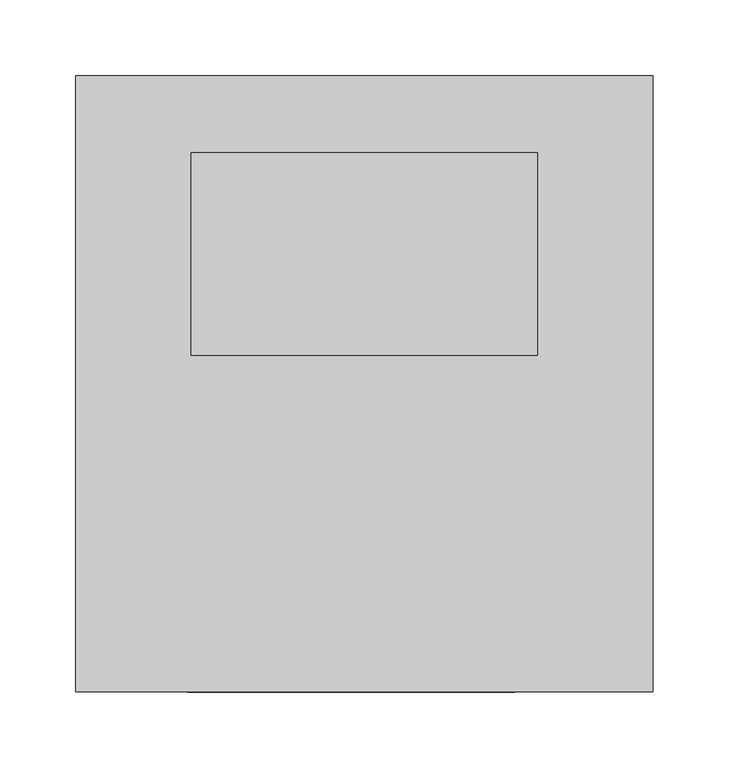
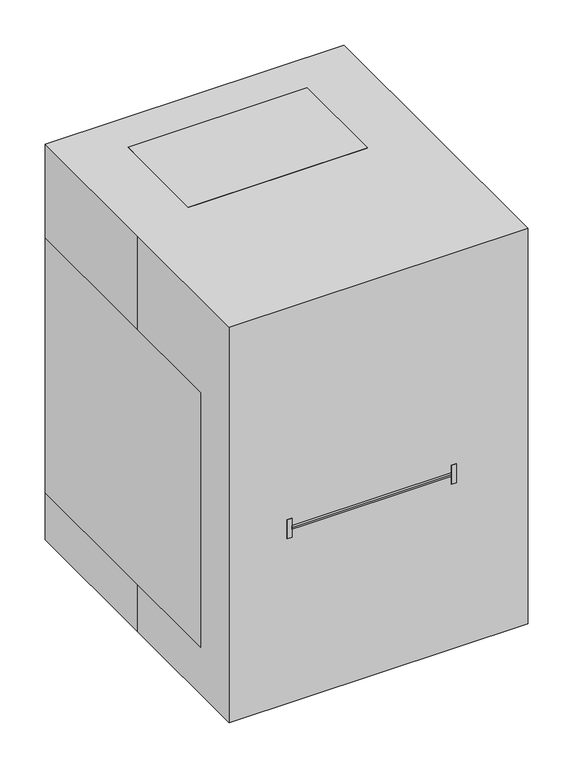
"""IFC4 building model written with IfcOpenShell, lengths in millimetres: proxy geometry, D4500 - Furnace, Laboratory, Dental, Burnout : D4500 - Furnace, Laboratory, Dental, Burnout."""

from ifc_helpers import new_model, si_unit, point, frame, frame_2d, origin, origin_with_axes, place, context, project, spatial, polyline, circle_curve, ellipse_curve, trimmed, segment, composite_curve, outline, extrude, source, transform, mapped, element, save
from ifc_brep_helpers import plane_surface, revolved_surface, advanced_brep


def specialty_equipment_c4cd605c(model_context):
    return source(origin(), model_context, "Body", "SolidModel", [
        extrude(outline(polyline([(0.0, -25.5914377), (0.0, 0.0), (12.6999999, 0.0), (12.6999999, -25.5914377), (0.0, -25.5914377)])), frame((58.817219, -9.8927789, 446.2580582), z_axis=(0.0, 0.18428853505018944, 0.9828721869343212), x_axis=(0.0, 0.9828721869343212, -0.18428853505018944)), (0.0, 0.0, 1.0), 12.7),
        extrude(outline(polyline([(0.0, -39.4493307), (0.0, 0.0), (12.7, 0.0), (12.7, -39.4493307), (0.0, -39.4493307)])), frame((58.817219, -5.1590339, 473.1988265), z_axis=(0.0, 0.18428853505018944, 0.9828721869343212), x_axis=(0.0, 0.9828721869343212, -0.18428853505018944)), (0.0, 0.0, 1.0), 12.7),
        advanced_brep(
        [(-33.7035425, 19.6808212, 515.5977131), (-61.832781, 19.6808212, 515.5977131), (-61.832781, 19.6808212, 502.8977131), (-33.7035425, 19.6808212, 502.8977131), (-33.7035425, 15.7120712, 515.5977131), (-61.832781, 15.7120712, 515.5977131), (-61.832781, 13.3308212, 502.8977131), (-33.7035425, 13.3308212, 502.8977131), (10.7464575, 19.6808212, 515.5977131), (-17.382781, 19.6808212, 515.5977131), (-17.382781, 19.6808212, 502.8977131), (10.7464575, 19.6808212, 502.8977131), (10.7464575, 15.7120712, 515.5977131), (-17.382781, 15.7120712, 515.5977131), (-17.382781, 13.3308212, 502.8977131), (10.7464575, 13.3308212, 502.8977131), (86.9464575, 19.6808212, 515.5977131), (58.817219, 19.6808212, 515.5977131), (58.817219, 19.6808212, 502.8977131), (86.9464575, 19.6808212, 502.8977131), (86.9464575, 15.7120712, 515.5977131), (58.817219, 15.7120712, 515.5977131), (58.817219, 13.3308212, 502.8977131), (86.9464575, 13.3308212, 502.8977131), (-81.3285425, 19.6808212, 515.5977131), (-98.425, 19.6808212, 515.5977131), (-98.425, 19.6808212, 502.8977131), (-81.3285425, 19.6808212, 502.8977131), (-81.3285425, 15.7120712, 515.5977131), (-98.425, 15.7120712, 515.5977131), (-98.425, 13.3308212, 502.8977131), (-81.3285425, 13.3308212, 502.8977131), (-1.1880744, 19.9716696, 476.932238), (11.5119256, 19.9716696, 476.932238), (-1.1880744, 8.4622946, 476.932238), (5.1619256, 7.2716696, 470.582238), (11.5119256, 8.4622946, 476.932238), (11.148763, 3.3029196, 449.4155713), (-0.8249118, 3.3029196, 449.4155713), (-1.1880744, 16.0029196, 451.532238), (11.5119256, 16.0029196, 451.532238), (-1.1880744, 3.6997946, 451.532238), (11.5119256, 3.6997946, 451.532238), (-13.5268228, 5.6841696, 462.1155713), (-19.8099793, 5.6841696, 462.1155713), (-23.0184011, 18.3841696, 467.6339938), (-10.3184011, 18.3841696, 467.6339938), (-23.0184011, 6.7188738, 467.6339938), (-10.3184011, 6.7188738, 467.6339938), (-38.9268228, 5.6841696, 462.1155713), (-45.2099793, 5.6841696, 462.1155713), (-48.4184011, 19.9716696, 467.6339938), (-35.7184011, 19.9716696, 467.6339938), (-48.4184011, 6.7188738, 467.6339938), (-35.7184011, 6.7188738, 467.6339938), (-64.3268228, 5.6841696, 462.1155713), (-70.6099793, 5.6841696, 462.1155713), (-73.8184011, 19.9716696, 467.6339938), (-61.1184011, 19.9716696, 467.6339938), (-73.8184011, 6.7188738, 467.6339938), (-61.1184011, 6.7188738, 467.6339938), (-86.5509752, 5.6841696, 462.1155713), (-92.8341316, 5.6841696, 462.1155713), (-96.0425534, 17.4344988, 467.6339938), (-83.3425534, 17.4344988, 467.6339938), (-96.0425534, 6.7188738, 467.6339938), (-83.3425534, 6.7188738, 467.6339938), (114.3, 152.4, 533.4), (-114.3, 152.4, 533.4), (-114.3, 19.05, 533.4), (114.3, 19.05, 533.4), (114.3, 152.4, 431.8), (114.3, 0.0, 431.8), (-114.3, 0.0, 431.8), (-114.3, 152.4, 431.8)],
        [
            (0, 1),
            (1, 2),
            (2, 3),
            (3, 0),
            (0, 4),
            (4, 5),
            (5, 1),
            (5, 6),
            (6, 2),
            (6, 7),
            (7, 3),
            (7, 4),
            (8, 9),
            (9, 10),
            (10, 11),
            (11, 8),
            (8, 12),
            (12, 13),
            (13, 9),
            (13, 14),
            (14, 10),
            (14, 15),
            (15, 11),
            (15, 12),
            (16, 17),
            (17, 18),
            (18, 19),
            (19, 16),
            (16, 20),
            (20, 21),
            (21, 17),
            (21, 22),
            (22, 18),
            (22, 23),
            (23, 19),
            (23, 20),
            (24, 25),
            (25, 26),
            (26, 27),
            (27, 24),
            (24, 28),
            (28, 29),
            (29, 25),
            (29, 30),
            (30, 26),
            (30, 31),
            (31, 27),
            (31, 28),
            (32, 33, circle_curve(frame((5.1619256, 19.9716696, 476.932238), z_axis=(0.0, -1.0, 0.0), x_axis=(1.0, 0.0, 0.0)), 6.35)),
            (33, 32, circle_curve(frame((5.1619256, 19.9716696, 476.932238), z_axis=(0.0, -1.0, 0.0), x_axis=(1.0, 0.0, 0.0)), 6.35)),
            (32, 34),
            (34, 35, ellipse_curve(frame((5.1619256, 8.4622946, 476.932238), z_axis=(0.0, -0.9828721869343219, 0.18428853505018564), x_axis=(0.0, -0.18428853505018514, -0.9828721869343221)), 6.4606569, 6.35)),
            (35, 36, ellipse_curve(frame((5.1619256, 8.4622946, 476.932238), z_axis=(0.0, -0.9828721869343219, 0.18428853505018564), x_axis=(0.0, -0.18428853505018514, -0.9828721869343221)), 6.4606569, 6.35)),
            (36, 33),
            (36, 34, ellipse_curve(frame((5.1619256, 8.4622946, 476.932238), z_axis=(0.0, -0.9828721869343219, 0.18428853505018564), x_axis=(0.0, -0.18428853505018514, -0.9828721869343221)), 6.4606569, 6.35)),
            (37, 38, circle_curve(frame((5.1619256, 3.3029196, 451.532238), z_axis=(0.0, 1.0, 0.0), x_axis=(1.0, 0.0, 0.0)), 6.35)),
            (38, 37),
            (39, 40, circle_curve(frame((5.1619256, 16.0029196, 451.532238), z_axis=(0.0, -1.0, 0.0), x_axis=(1.0, 0.0, 0.0)), 6.35)),
            (40, 39, circle_curve(frame((5.1619256, 16.0029196, 451.532238), z_axis=(0.0, -1.0, 0.0), x_axis=(1.0, 0.0, 0.0)), 6.35)),
            (39, 41),
            (41, 38, ellipse_curve(frame((5.1619256, 3.6997946, 451.532238), z_axis=(0.0, -0.9828721869343219, 0.18428853505018564), x_axis=(0.0, -0.18428853505018514, -0.9828721869343221)), 6.4606569, 6.35)),
            (37, 42, ellipse_curve(frame((5.1619256, 3.6997946, 451.532238), z_axis=(0.0, -0.9828721869343219, 0.18428853505018564), x_axis=(0.0, -0.18428853505018514, -0.9828721869343221)), 6.4606569, 6.35)),
            (42, 40),
            (42, 41, ellipse_curve(frame((5.1619256, 3.6997946, 451.532238), z_axis=(0.0, -0.9828721869343219, 0.18428853505018564), x_axis=(0.0, -0.18428853505018514, -0.9828721869343221)), 6.4606569, 6.35)),
            (43, 44, circle_curve(frame((-16.6684011, 5.6841696, 467.6339938), z_axis=(0.0, 1.0, 0.0), x_axis=(1.0, 0.0, 0.0)), 6.35)),
            (44, 43),
            (45, 46, circle_curve(frame((-16.6684011, 18.3841696, 467.6339938), z_axis=(0.0, -1.0, 0.0), x_axis=(1.0, 0.0, 0.0)), 6.35)),
            (46, 45, circle_curve(frame((-16.6684011, 18.3841696, 467.6339938), z_axis=(0.0, -1.0, 0.0), x_axis=(1.0, 0.0, 0.0)), 6.35)),
            (45, 47),
            (47, 44, ellipse_curve(frame((-16.6684011, 6.7188738, 467.6339938), z_axis=(0.0, -0.9828721869343219, 0.18428853505018564), x_axis=(0.0, -0.18428853505018514, -0.9828721869343221)), 6.4606569, 6.35)),
            (43, 48, ellipse_curve(frame((-16.6684011, 6.7188738, 467.6339938), z_axis=(0.0, -0.9828721869343219, 0.18428853505018564), x_axis=(0.0, -0.18428853505018514, -0.9828721869343221)), 6.4606569, 6.35)),
            (48, 46),
            (48, 47, ellipse_curve(frame((-16.6684011, 6.7188738, 467.6339938), z_axis=(0.0, -0.9828721869343219, 0.18428853505018564), x_axis=(0.0, -0.18428853505018514, -0.9828721869343221)), 6.4606569, 6.35)),
            (49, 50, circle_curve(frame((-42.0684011, 5.6841696, 467.6339938), z_axis=(0.0, 1.0, 0.0), x_axis=(1.0, 0.0, 0.0)), 6.35)),
            (50, 49),
            (51, 52, circle_curve(frame((-42.0684011, 19.9716696, 467.6339938), z_axis=(0.0, -1.0, 0.0), x_axis=(1.0, 0.0, 0.0)), 6.35)),
            (52, 51, circle_curve(frame((-42.0684011, 19.9716696, 467.6339938), z_axis=(0.0, -1.0, 0.0), x_axis=(1.0, 0.0, 0.0)), 6.35)),
            (51, 53),
            (53, 50, ellipse_curve(frame((-42.0684011, 6.7188738, 467.6339938), z_axis=(0.0, -0.9828721869343219, 0.18428853505018564), x_axis=(0.0, -0.18428853505018514, -0.9828721869343221)), 6.4606569, 6.35)),
            (49, 54, ellipse_curve(frame((-42.0684011, 6.7188738, 467.6339938), z_axis=(0.0, -0.9828721869343219, 0.18428853505018564), x_axis=(0.0, -0.18428853505018514, -0.9828721869343221)), 6.4606569, 6.35)),
            (54, 52),
            (54, 53, ellipse_curve(frame((-42.0684011, 6.7188738, 467.6339938), z_axis=(0.0, -0.9828721869343219, 0.18428853505018564), x_axis=(0.0, -0.18428853505018514, -0.9828721869343221)), 6.4606569, 6.35)),
            (55, 56, circle_curve(frame((-67.4684011, 5.6841696, 467.6339938), z_axis=(0.0, 1.0, 0.0), x_axis=(1.0, 0.0, 0.0)), 6.35)),
            (56, 55),
            (57, 58, circle_curve(frame((-67.4684011, 19.9716696, 467.6339938), z_axis=(0.0, -1.0, 0.0), x_axis=(1.0, 0.0, 0.0)), 6.35)),
            (58, 57, circle_curve(frame((-67.4684011, 19.9716696, 467.6339938), z_axis=(0.0, -1.0, 0.0), x_axis=(1.0, 0.0, 0.0)), 6.35)),
            (57, 59),
            (59, 56, ellipse_curve(frame((-67.4684011, 6.7188738, 467.6339938), z_axis=(0.0, -0.9828721869343219, 0.18428853505018564), x_axis=(0.0, -0.18428853505018514, -0.9828721869343221)), 6.4606569, 6.35)),
            (55, 60, ellipse_curve(frame((-67.4684011, 6.7188738, 467.6339938), z_axis=(0.0, -0.9828721869343219, 0.18428853505018564), x_axis=(0.0, -0.18428853505018514, -0.9828721869343221)), 6.4606569, 6.35)),
            (60, 58),
            (60, 59, ellipse_curve(frame((-67.4684011, 6.7188738, 467.6339938), z_axis=(0.0, -0.9828721869343219, 0.18428853505018564), x_axis=(0.0, -0.18428853505018514, -0.9828721869343221)), 6.4606569, 6.35)),
            (61, 62, circle_curve(frame((-89.6925534, 5.6841696, 467.6339938), z_axis=(0.0, 1.0, 0.0), x_axis=(1.0, 0.0, 0.0)), 6.35)),
            (62, 61),
            (63, 64, circle_curve(frame((-89.6925534, 17.4344988, 467.6339938), z_axis=(0.0, -1.0, 0.0), x_axis=(1.0, 0.0, 0.0)), 6.35)),
            (64, 63, circle_curve(frame((-89.6925534, 17.4344988, 467.6339938), z_axis=(0.0, -1.0, 0.0), x_axis=(1.0, 0.0, 0.0)), 6.35)),
            (63, 65),
            (65, 62, ellipse_curve(frame((-89.6925534, 6.7188738, 467.6339938), z_axis=(0.0, -0.9828721869343219, 0.18428853505018564), x_axis=(0.0, -0.18428853505018514, -0.9828721869343221)), 6.4606569, 6.35)),
            (61, 66, ellipse_curve(frame((-89.6925534, 6.7188738, 467.6339938), z_axis=(0.0, -0.9828721869343219, 0.18428853505018564), x_axis=(0.0, -0.18428853505018514, -0.9828721869343221)), 6.4606569, 6.35)),
            (66, 64),
            (66, 65, ellipse_curve(frame((-89.6925534, 6.7188738, 467.6339938), z_axis=(0.0, -0.9828721869343219, 0.18428853505018564), x_axis=(0.0, -0.18428853505018514, -0.9828721869343221)), 6.4606569, 6.35)),
            (67, 68),
            (68, 69),
            (69, 70),
            (70, 67),
            (71, 72),
            (72, 73),
            (73, 74),
            (74, 71),
            (67, 71),
            (74, 68),
            (73, 69),
            (72, 70),
        ],
        [
            plane_surface(frame((-61.832781, 19.6808212, 515.5977131), z_axis=(0.0, -1.0, 0.0), x_axis=(1.0, 0.0, 0.0))),
            plane_surface(frame((-33.7035425, 13.3308212, 515.5977131), z_axis=(0.0, 0.0, -1.0), x_axis=(0.0, 1.0, 0.0))),
            plane_surface(frame((-61.832781, 13.3308212, 515.5977131), z_axis=(1.0, 0.0, 0.0), x_axis=(0.0, 1.0, 0.0))),
            plane_surface(frame((-61.832781, 13.3308212, 502.8977131), z_axis=(0.0, 0.0, 1.0), x_axis=(0.0, 1.0, 0.0))),
            plane_surface(frame((-33.7035425, 13.3308212, 502.8977131), z_axis=(-1.0, 0.0, 0.0), x_axis=(0.0, 1.0, 0.0))),
            plane_surface(frame((-17.382781, 19.6808212, 515.5977131), z_axis=(0.0, -1.0, 0.0), x_axis=(1.0, 0.0, 0.0))),
            plane_surface(frame((10.7464575, 13.3308212, 515.5977131), z_axis=(0.0, 0.0, -1.0), x_axis=(0.0, 1.0, 0.0))),
            plane_surface(frame((-17.382781, 13.3308212, 515.5977131), z_axis=(1.0, 0.0, 0.0), x_axis=(0.0, 1.0, 0.0))),
            plane_surface(frame((-17.382781, 13.3308212, 502.8977131), z_axis=(0.0, 0.0, 1.0), x_axis=(0.0, 1.0, 0.0))),
            plane_surface(frame((10.7464575, 13.3308212, 502.8977131), z_axis=(-1.0, 0.0, 0.0), x_axis=(0.0, 1.0, 0.0))),
            plane_surface(frame((58.817219, 19.6808212, 515.5977131), z_axis=(0.0, -1.0, 0.0), x_axis=(1.0, 0.0, 0.0))),
            plane_surface(frame((86.9464575, 13.3308212, 515.5977131), z_axis=(0.0, 0.0, -1.0), x_axis=(0.0, 1.0, 0.0))),
            plane_surface(frame((58.817219, 13.3308212, 515.5977131), z_axis=(1.0, 0.0, 0.0), x_axis=(0.0, 1.0, 0.0))),
            plane_surface(frame((58.817219, 13.3308212, 502.8977131), z_axis=(0.0, 0.0, 1.0), x_axis=(0.0, 1.0, 0.0))),
            plane_surface(frame((86.9464575, 13.3308212, 502.8977131), z_axis=(-1.0, 0.0, 0.0), x_axis=(0.0, 1.0, 0.0))),
            plane_surface(frame((-109.457781, 19.6808212, 515.5977131), z_axis=(0.0, -1.0, 0.0), x_axis=(1.0, 0.0, 0.0))),
            plane_surface(frame((-81.3285425, 13.3308212, 515.5977131), z_axis=(0.0, 0.0, -1.0), x_axis=(0.0, 1.0, 0.0))),
            plane_surface(frame((-98.425, 13.3308212, 515.5977131), z_axis=(1.0, 0.0, 0.0), x_axis=(0.0, 1.0, 0.0))),
            plane_surface(frame((-98.425, 13.3308212, 502.8977131), z_axis=(0.0, 0.0, 1.0), x_axis=(0.0, 1.0, 0.0))),
            plane_surface(frame((-81.3285425, 13.3308212, 502.8977131), z_axis=(-1.0, 0.0, 0.0), x_axis=(0.0, 1.0, 0.0))),
            plane_surface(frame((11.5119256, 19.9716696, 476.932238), z_axis=(0.0, -1.0, 0.0), x_axis=(0.0, 0.0, -1.0))),
            revolved_surface(polyline([(11.5119256, 7.271669599999999, 476.932238), (11.5119256, 19.9716696, 476.932238)]), (5.1619256, 19.9716696, 476.932238), (0.0, -1.0, 0.0)),
            revolved_surface(polyline([(11.5119256, 7.271669604437129, 476.932238), (11.5119256, 19.9716696, 476.932238)]), (5.1619256, 19.9716696, 476.932238), (0.0, -1.0, 0.0)),
            plane_surface(frame((11.5119256, 3.3029196, 451.532238), z_axis=(0.0, 1.0, 0.0), x_axis=(0.0, 0.0, 1.0))),
            plane_surface(frame((11.5119256, 16.0029196, 451.532238), z_axis=(0.0, -1.0, 0.0), x_axis=(0.0, 0.0, -1.0))),
            revolved_surface(polyline([(11.5119256, 2.5091696044371297, 451.532238), (11.5119256, 16.0029196, 451.532238)]), (5.1619256, 16.0029196, 451.532238), (0.0, -1.0, 0.0)),
            plane_surface(frame((-10.3184011, 5.6841696, 467.6339938), z_axis=(0.0, 1.0, 0.0), x_axis=(0.0, 0.0, 1.0))),
            plane_surface(frame((-10.3184011, 18.3841696, 467.6339938), z_axis=(0.0, -1.0, 0.0), x_axis=(0.0, 0.0, -1.0))),
            revolved_surface(polyline([(-10.3184011, 5.52824880443713, 467.6339938), (-10.3184011, 18.3841696, 467.6339938)]), (-16.6684011, 18.3841696, 467.6339938), (0.0, -1.0, 0.0)),
            plane_surface(frame((-35.7184011, 5.6841696, 467.6339938), z_axis=(0.0, 1.0, 0.0), x_axis=(0.0, 0.0, 1.0))),
            plane_surface(frame((-35.7184011, 19.9716696, 467.6339938), z_axis=(0.0, -1.0, 0.0), x_axis=(0.0, 0.0, -1.0))),
            revolved_surface(polyline([(-35.7184011, 5.52824880443713, 467.6339938), (-35.7184011, 19.9716696, 467.6339938)]), (-42.0684011, 19.9716696, 467.6339938), (0.0, -1.0, 0.0)),
            plane_surface(frame((-61.1184011, 5.6841696, 467.6339938), z_axis=(0.0, 1.0, 0.0), x_axis=(0.0, 0.0, 1.0))),
            plane_surface(frame((-61.1184011, 19.9716696, 467.6339938), z_axis=(0.0, -1.0, 0.0), x_axis=(0.0, 0.0, -1.0))),
            revolved_surface(polyline([(-61.11840109999999, 5.52824880443713, 467.6339938), (-61.11840109999999, 19.9716696, 467.6339938)]), (-67.4684011, 19.9716696, 467.6339938), (0.0, -1.0, 0.0)),
            plane_surface(frame((-83.3425534, 5.6841696, 467.6339938), z_axis=(0.0, 1.0, 0.0), x_axis=(0.0, 0.0, 1.0))),
            plane_surface(frame((-83.3425534, 17.4344988, 467.6339938), z_axis=(0.0, -1.0, 0.0), x_axis=(0.0, 0.0, -1.0))),
            revolved_surface(polyline([(-83.3425534, 5.52824880443713, 467.6339938), (-83.3425534, 17.4344988, 467.6339938)]), (-89.6925534, 17.4344988, 467.6339938), (0.0, -1.0, 0.0)),
            plane_surface(frame((0.0, 85.725, 533.4), z_axis=(0.0, 0.0, 1.0), x_axis=(-1.0, 0.0, 0.0))),
            plane_surface(frame((0.0, 76.2, 431.8), z_axis=(0.0, 0.0, -1.0), x_axis=(-1.0, 0.0, 0.0))),
            plane_surface(frame((0.0, 152.4, 431.8), z_axis=(0.0, 1.0, 0.0), x_axis=(-1.0, 0.0, 0.0))),
            plane_surface(frame((-114.3, 76.2, 431.8), z_axis=(-1.0, 0.0, 0.0), x_axis=(0.0, -1.0, 0.0))),
            plane_surface(frame((0.0, 0.0, 431.8), z_axis=(0.0, -0.9828721869343219, 0.18428853505018564), x_axis=(1.0, 0.0, 0.0))),
            plane_surface(frame((114.3, 76.2, 431.8), z_axis=(1.0, 0.0, 0.0), x_axis=(0.0, 1.0, 0.0))),
        ],
        [
            (0, [[1, 2, 3, 4]]),
            (1, [[-1, 5, 6, 7]]),
            (2, [[-2, -7, 8, 9]]),
            (3, [[-3, -9, 10, 11]]),
            (4, [[-4, -11, 12, -5]]),
            (5, [[13, 14, 15, 16]]),
            (6, [[-13, 17, 18, 19]]),
            (7, [[-14, -19, 20, 21]]),
            (8, [[-15, -21, 22, 23]]),
            (9, [[-16, -23, 24, -17]]),
            (10, [[25, 26, 27, 28]]),
            (11, [[-25, 29, 30, 31]]),
            (12, [[-26, -31, 32, 33]]),
            (13, [[-27, -33, 34, 35]]),
            (14, [[-28, -35, 36, -29]]),
            (15, [[37, 38, 39, 40]]),
            (16, [[-37, 41, 42, 43]]),
            (17, [[-38, -43, 44, 45]]),
            (18, [[-39, -45, 46, 47]]),
            (19, [[-40, -47, 48, -41]]),
            (20, [[49, 50]]),
            (21, [[-49, 51, 52, 53, 54]]),
            (22, [[-50, -54, 55, -51]]),
            (23, [[56, 57]]),
            (24, [[58, 59]]),
            (25, [[-58, 60, 61, -56, 62, 63]]),
            (25, [[-59, -63, 64, -60]]),
            (26, [[65, 66]]),
            (27, [[67, 68]]),
            (28, [[-67, 69, 70, -65, 71, 72]]),
            (28, [[-68, -72, 73, -69]]),
            (29, [[74, 75]]),
            (30, [[76, 77]]),
            (31, [[-76, 78, 79, -74, 80, 81]]),
            (31, [[-77, -81, 82, -78]]),
            (32, [[83, 84]]),
            (33, [[85, 86]]),
            (34, [[-85, 87, 88, -83, 89, 90]]),
            (34, [[-86, -90, 91, -87]]),
            (35, [[92, 93]]),
            (36, [[94, 95]]),
            (37, [[-94, 96, 97, -92, 98, 99]]),
            (37, [[-95, -99, 100, -96]]),
            (38, [[101, 102, 103, 104]]),
            (39, [[105, 106, 107, 108]]),
            (40, [[-101, 109, -108, 110]]),
            (41, [[-102, -110, -107, 111]]),
            (42, [[-103, -111, -106, 112], [-6, -12, -10, -8], [-18, -24, -22, -20], [-30, -36, -34, -32], [-42, -48, -46, -44], [-53, -52, -55], [-75, -79, -82, -80], [-84, -88, -91, -89], [-57, -61, -64, -62], [-93, -97, -100, -98], [-66, -70, -73, -71]]),
            (43, [[-104, -112, -105, -109]]),
        ],
    ),
        extrude(outline(polyline([(0.0, 140.2685872), (0.0, 165.6685872), (63.5, 165.6685872), (63.5, 127.5685872), (0.0, 140.2685872)])), frame((0.0, 139.7, 0.0), z_axis=(0.0, 1.0, 0.0), x_axis=(0.0, 0.0, 1.0)), (0.0, 0.0, 1.0), 38.1),
        extrude(outline(polyline([(0.0, -165.6685872), (0.0, -140.2685872), (63.5, -127.5685872), (63.5, -165.6685872), (0.0, -165.6685872)])), frame((0.0, 139.7, 0.0), z_axis=(0.0, 1.0, 0.0), x_axis=(0.0, 0.0, 1.0)), (0.0, 0.0, 1.0), 38.1),
        extrude(outline(polyline([(0.0, 140.2685872), (0.0, 165.6685872), (63.5, 165.6685872), (63.5, 127.5685872), (0.0, 140.2685872)])), frame((0.0, -114.3, 0.0), z_axis=(0.0, 1.0, 0.0), x_axis=(0.0, 0.0, 1.0)), (0.0, 0.0, 1.0), 38.1),
        extrude(outline(polyline([(0.0, -165.6685872), (0.0, -140.2685872), (63.5, -127.5685872), (63.5, -165.6685872), (0.0, -165.6685872)])), frame((0.0, -114.3, 0.0), z_axis=(0.0, 1.0, 0.0), x_axis=(0.0, 0.0, 1.0)), (0.0, 0.0, 1.0), 38.1),
        extrude(outline(composite_curve([segment(trimmed(circle_curve(frame_2d((-137.0420305, -146.8558318)), 6.35), [point((-137.0420305, -140.5058318))], [point((-137.0420305, -153.2058318))], False, "CARTESIAN"), True, "CONTINUOUS"), segment(trimmed(circle_curve(frame_2d((-137.0420305, -146.8558318)), 6.35), [point((-137.0420305, -153.2058318))], [point((-137.0420305, -140.5058318))], False, "CARTESIAN"), True, "CONTINUOUS")], self_intersect=False)), frame((0.0, 0.0, 81.7902562), z_axis=(0.0, 0.0, 1.0), x_axis=(1.0, 0.0, 0.0)), (0.0, 0.0, 1.0), 25.6207018),
        extrude(outline(composite_curve([segment(trimmed(circle_curve(frame_2d((-10.0420305, -157.9683318)), 6.35), [point((-10.0420305, -151.6183318))], [point((-10.0420305, -164.3183318))], False, "CARTESIAN"), True, "CONTINUOUS"), segment(trimmed(circle_curve(frame_2d((-10.0420305, -157.9683318)), 6.35), [point((-10.0420305, -164.3183318))], [point((-10.0420305, -151.6183318))], False, "CARTESIAN"), True, "CONTINUOUS")], self_intersect=False)), frame((0.0, 0.0, 82.144649), z_axis=(0.0, 0.0, 1.0), x_axis=(1.0, 0.0, 0.0)), (0.0, 0.0, 1.0), 31.6831545),
        extrude(outline(polyline([(-10.31875, -161.13125), (-134.439745, -150.27207), (-133.8863061, -143.9462337), (-9.765311, -154.8054137), (-10.31875, -161.13125)])), frame((0.0, 0.0, 88.494649), z_axis=(0.0, 0.0, 1.0), x_axis=(1.0, 0.0, 0.0)), (0.0, 0.0, 1.0), 12.7),
        extrude(outline(composite_curve([segment(trimmed(circle_curve(frame_2d((-137.0420305, -146.8558318)), 6.35), [point((-143.3920305, -146.8558318))], [point((-130.6920305, -146.8558318))], False, "CARTESIAN"), True, "CONTINUOUS"), segment(trimmed(circle_curve(frame_2d((-137.0420305, -146.8558318)), 6.35), [point((-130.6920305, -146.8558318))], [point((-143.3920305, -146.8558318))], False, "CARTESIAN"), True, "CONTINUOUS")], self_intersect=False)), frame((0.0, 0.0, 362.1346492), z_axis=(0.0, 0.0, 1.0), x_axis=(1.0, 0.0, 0.0)), (0.0, 0.0, 1.0), 25.6207018),
        extrude(outline(composite_curve([segment(trimmed(circle_curve(frame_2d((-10.0420305, -157.9683318)), 6.35), [point((-16.3920305, -157.9683318))], [point((-3.6920305, -157.9683318))], False, "CARTESIAN"), True, "CONTINUOUS"), segment(trimmed(circle_curve(frame_2d((-10.0420305, -157.9683318)), 6.35), [point((-3.6920305, -157.9683318))], [point((-16.3920305, -157.9683318))], False, "CARTESIAN"), True, "CONTINUOUS")], self_intersect=False)), frame((0.0, 0.0, 356.0721965), z_axis=(0.0, 0.0, 1.0), x_axis=(1.0, 0.0, 0.0)), (0.0, 0.0, 1.0), 31.6831545),
        extrude(outline(polyline([(-10.31875, -161.13125), (-134.439745, -150.27207), (-133.8863061, -143.9462337), (-9.765311, -154.8054137), (-10.31875, -161.13125)])), frame((0.0, 0.0, 368.705351), z_axis=(0.0, 0.0, 1.0), x_axis=(1.0, 0.0, 0.0)), (0.0, 0.0, 1.0), 12.7),
        extrude(outline(composite_curve([segment(trimmed(circle_curve(frame_2d((-193.7562446, 234.95)), 9.4798715), [point((-203.2361161, 234.95))], [point((-184.2763731, 234.95))], False, "CARTESIAN"), True, "CONTINUOUS"), segment(trimmed(circle_curve(frame_2d((-193.7562446, 234.95)), 9.4798715), [point((-184.2763731, 234.95))], [point((-203.2361161, 234.95))], False, "CARTESIAN"), True, "CONTINUOUS")], self_intersect=False)), frame((-110.2767662, 0.0, 0.0), z_axis=(1.0, 0.0, 0.0), x_axis=(0.0, 1.0, 0.0)), (0.0, 0.0, 1.0), 203.2),
        extrude(outline(polyline([(-110.2767662, -139.7361161), (-110.2767662, -203.2361161), (-116.6267662, -203.2361161), (-116.6267662, -139.7361161), (-110.2767662, -139.7361161)])), frame((0.0, 0.0, 222.25), z_axis=(0.0, 0.0, 1.0), x_axis=(1.0, 0.0, 0.0)), (0.0, 0.0, 1.0), 25.4),
        extrude(outline(polyline([(99.2732338, -139.7361161), (99.2732338, -203.2361161), (92.9232338, -203.2361161), (92.9232338, -139.7361161), (99.2732338, -139.7361161)])), frame((0.0, 0.0, 222.25), z_axis=(0.0, 0.0, 1.0), x_axis=(1.0, 0.0, 0.0)), (0.0, 0.0, 1.0), 25.4),
        extrude(outline(polyline([(92.9232338, -139.7), (92.9232338, -165.1), (-110.2767662, -165.1), (-110.2767662, -139.7), (92.9232338, -139.7)])), frame((0.0, 0.0, 113.8278035), z_axis=(0.0, 0.0, 1.0), x_axis=(1.0, 0.0, 0.0)), (0.0, 0.0, 1.0), 242.244393),
        extrude(outline(polyline([(190.5, 203.2), (190.5, -139.7), (-190.5, -139.7), (-190.5, 203.2), (190.5, 203.2)])), frame((0.0, 0.0, 63.5), z_axis=(0.0, 0.0, 1.0), x_axis=(1.0, 0.0, 0.0)), (0.0, 0.0, 1.0), 342.9),
        extrude(outline(polyline([(95.25, 25.4), (-95.25, 25.4), (-95.25, 127.0), (95.25, 127.0), (95.25, 25.4)])), frame((0.0, 0.0, 406.4), z_axis=(0.0, 0.0, 1.0), x_axis=(1.0, 0.0, 0.0)), (0.0, 0.0, 1.0), 25.4),
        extrude(outline(polyline([(-190.5, 203.2), (190.5, 203.2), (190.5, -203.2), (-190.5, -203.2), (-190.5, 0.0), (-190.5, 203.2)])), origin_with_axes(), (0.0, 0.0, 1.0), 533.4),
    ])


if __name__ == "__main__":
    model = new_model("IFC4")
    model_context = context("Model", 3, world=origin())
    ifc_project = project(units=[si_unit("LENGTHUNIT", "METRE", prefix="MILLI")], contexts=[model_context])
    site = spatial("IfcSite", under=ifc_project)
    building = spatial("IfcBuilding", under=site)
    placement = place(None, origin())
    specialty_equipment_shape = specialty_equipment_c4cd605c(model_context)
    element("IfcBuildingElementProxy", 1, Name="D4500 - Furnace, Laboratory, Dental, Burnout : D4500 - Furnace, Laboratory, Dental, Burnout", ObjectType="D4500 - Furnace, Laboratory, Dental, Burnout : D4500 - Furnace, Laboratory, Dental, Burnout", at=placement, inside=building, context=model_context, shape_type="MappedRepresentation", body=[
        mapped(specialty_equipment_shape, transform((0.0, 0.0, 0.0), x_axis=(1.0, 0.0, 0.0), y_axis=(0.0, 1.0, 0.0), z_axis=(0.0, 0.0, 1.0))),
    ])
    save(model, "model.ifc")

# Revit data of these elements
# Type "D4500 - Furnace, Laboratory, Dental, Burnout : D4500 - Furnace, Laboratory, Dental, Burnout"
#   Watts2 = "0"
#   Watts1 = "1400"
#   Unit_Issue = "EA"
#   UTIL_6_Misc = "-"
#   UTIL_5_NonMedGas = "-"
#   UTIL_4_MiscGas = "-"
#   UTIL_3_MedGas = "-"
#   UTIL_2_Elec = "A"
#   UTIL_1_WaterDrain = "-"
#   Nomenclature = "Furnace, Laboratory, Dental, Burnout"
#   NSN = "6520012558162"
#   Location [instance default] = ""
#   JSN = "D4500"
#   Fund_Source_VA = "-"
#   Fund_Source_Navy = "-"
#   Fund_Source_Army = "-"
#   Fund_Source_AF = "-"
#   ELEC_Volts2 = "0"
#   ELEC_Volts1 = "120"
#   ELEC_Phase2 = "0"
#   ELEC_Phase1 = "1"
#   ELEC_HertzSwitch = "0"
#   ELEC_HertzDependent = "-1"
#   ELEC_Hertz = "60"
#   ELEC_Amps2 = "0"
#   ELEC_Amps1 = "12"
#   DetailDescription = "Dental burnout furnace. The unit is used in dental laboratories for burnout of dental alloy rings and flasks. The furnace is capable of automatic or manual operation and has a automatic self-calibration system as well as a digital readout. The unit can hold a minimum of fifteen 1-3/4\" inlay rings. Some model lines are available with several sizes of heating elements and/or for other power configurations."
#   CAT_VA = "C"
#   CAT_Navy = "C"
#   CAT_IHS = "-"
#   CAT_Army = "C"
#   CAT_AF = "C"
#   BTUperhour = "0"
#   Weight_IP = 59
#   DIM_Width_IP = 1' - 3"
#   DIM_Height_IP = 1' - 9"
#   DIM_Depth_IP = 1' - 4"
# Element 1 (IfcBuildingElementProxy, "D4500 - Furnace, Laboratory, Dental, Burnout : D4500 - Furnace, Laboratory, Dental, Burnout")
#   Materials on its faces: "EquipSpace"
# Materials
#   "EquipSpace": class "Unassigned", colour RGB 221 217 195, transparency 0.5
